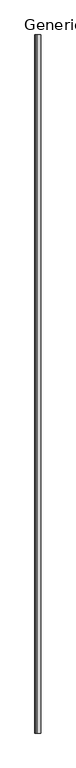
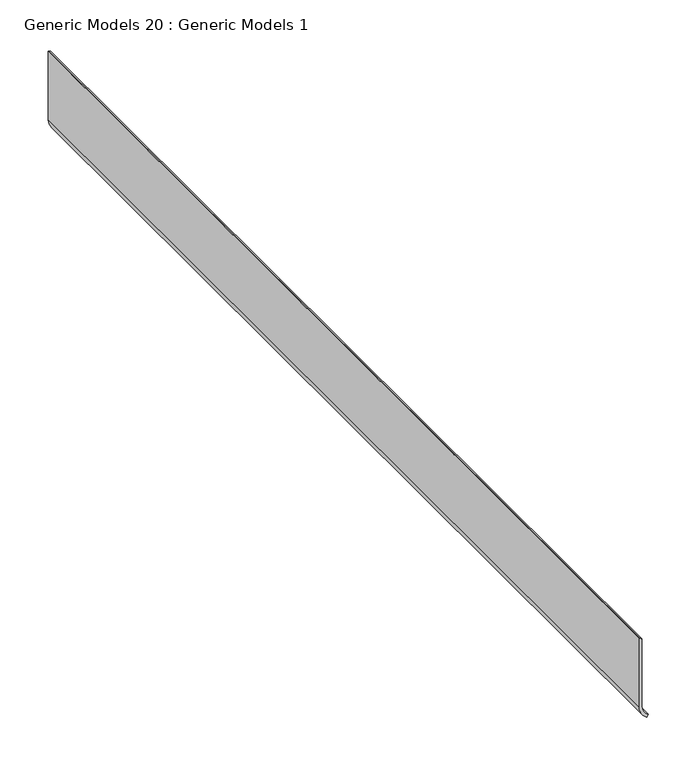
"""IFC4 building model written with IfcOpenShell, lengths in millimetres: proxy geometry, Generic Models 20 : Generic Models 1."""

from ifc_helpers import new_model, si_unit, point, frame, frame_2d, origin, place, context, project, spatial, polyline, circle_curve, trimmed, segment, composite_curve, outline, extrude, source, transform, mapped, element, save


def generic_models_20_generic_models_1_59b4b801(model_context):
    return source(origin(), model_context, "Body", "SweptSolid", [
        extrude(outline(composite_curve([segment(polyline([(73.749588, 51108.5310187), (-12.4007813, 51108.5310187)]), True, "CONTINUOUS"), segment(trimmed(circle_curve(frame_2d((-12.4007813, 51126.3707155)), 17.8396968), [point((-12.4007813, 51108.5310187))], [point((-27.850412, 51117.4508671))], False, "CARTESIAN"), True, "CONTINUOUS"), segment(polyline([(-27.850412, 51117.4508671), (-25.1007813, 51119.0383671)]), True, "CONTINUOUS"), segment(trimmed(circle_curve(frame_2d((-12.4007813, 51126.3707155)), 14.6646968), [point((-25.1007813, 51119.0383671))], [point((-12.4007813, 51111.7060187))], True, "CARTESIAN"), True, "CONTINUOUS"), segment(polyline([(-12.4007813, 51111.7060187), (71.6627862, 51111.7060187)]), True, "CONTINUOUS"), segment(trimmed(circle_curve(frame_2d((71.6627862, 51109.6192169)), 2.0868018), [point((71.6627862, 51111.7060187))], [point((73.749588, 51109.6192169))], False, "CARTESIAN"), True, "CONTINUOUS"), segment(polyline([(73.749588, 51109.6192169), (73.749588, 51108.5310187)]), True, "CONTINUOUS")], self_intersect=False)), frame((0.0, 0.0, 0.0), z_axis=(0.0, 1.0, 0.0), x_axis=(0.0, 0.0, 1.0)), (0.0, 0.0, 1.0), 1219.2),
    ])


if __name__ == "__main__":
    model = new_model("IFC4")
    model_context = context("Model", 3, world=origin())
    ifc_project = project(units=[si_unit("LENGTHUNIT", "METRE", prefix="MILLI")], contexts=[model_context])
    site = spatial("IfcSite", under=ifc_project)
    building = spatial("IfcBuilding", under=site)
    placement = place(None, origin())
    generic_models_20_generic_models_1_shape = generic_models_20_generic_models_1_59b4b801(model_context)
    element("IfcBuildingElementProxy", 1, Name="Generic Models 20 : Generic Models 1", ObjectType="Generic Models 20 : Generic Models 1", at=placement, inside=building, context=model_context, shape_type="MappedRepresentation", body=[
        mapped(generic_models_20_generic_models_1_shape, transform((0.0, 0.0, 0.0), x_axis=(1.0, 0.0, 0.0), y_axis=(0.0, 1.0, 0.0), z_axis=(0.0, 0.0, 1.0))),
    ])
    save(model, "model.ifc")

# Revit data of these elements
# Element 1 (IfcBuildingElementProxy, "Generic Models 20 : Generic Models 1")
#   Materials on its faces: "BASE AS SCHEDULED"
# Materials
#   "BASE AS SCHEDULED": class "Generic", colour RGB 120 120 120, transparency 0, Cost = 0
